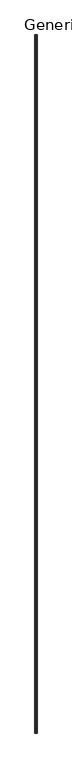
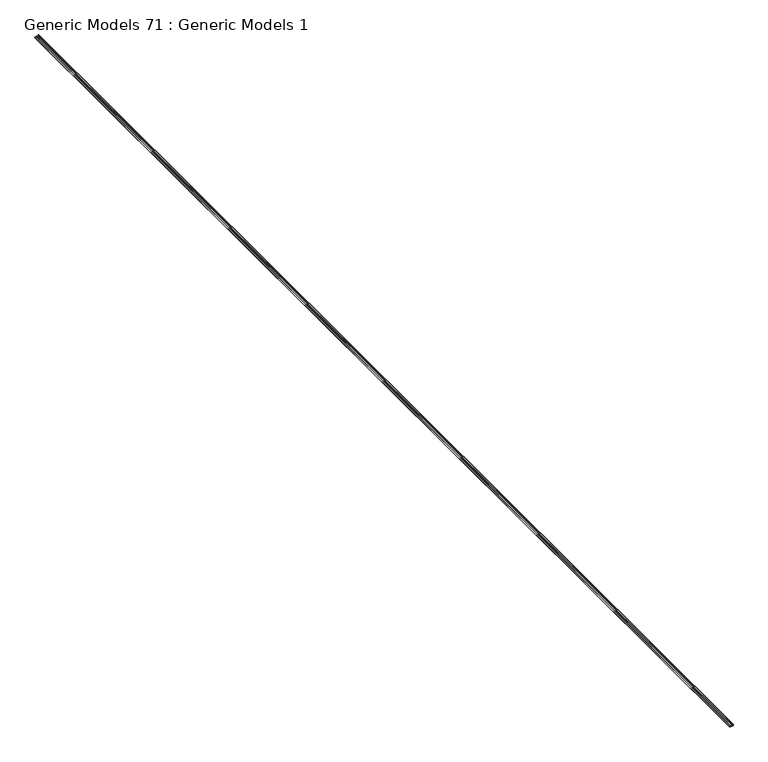
"""IFC4 building model written with IfcOpenShell, lengths in millimetres: proxy geometry, Generic Models 71 : Generic Models 1."""

from ifc_helpers import new_model, si_unit, frame, origin, place, context, project, spatial, polyline, outline, extrude, source, transform, mapped, element, save


def generic_models_71_generic_models_1_deb8e508(model_context):
    return source(origin(), model_context, "Body", "SweptSolid", [
        extrude(outline(polyline([(142822.070303, -9211.2597887), (142822.070303, -9230.9447887), (142833.500303, -9230.9447887), (142833.500303, -9246.1847887), (142822.070303, -9246.1847887), (142822.070303, -9268.6279726), (142820.800303, -9268.6279726), (142820.800303, -9244.9147887), (142832.230303, -9244.9147887), (142832.230303, -9232.2147887), (142820.800303, -9232.2147887), (142820.800303, -9209.9897887), (142825.550103, -9209.9897887), (142825.550103, -9210.8486296), (142844.5946817, -9210.8486296), (142844.5946817, -9212.1186296), (142824.280103, -9212.1186296), (142824.280103, -9211.2597887), (142822.070303, -9211.2597887)])), frame((0.0, -7068.1230338, 0.0), z_axis=(0.0, 1.0, 0.0), x_axis=(0.0, 0.0, 1.0)), (0.0, 0.0, 1.0), 19050.0),
    ])


if __name__ == "__main__":
    model = new_model("IFC4")
    model_context = context("Model", 3, world=origin())
    ifc_project = project(units=[si_unit("LENGTHUNIT", "METRE", prefix="MILLI")], contexts=[model_context])
    site = spatial("IfcSite", under=ifc_project)
    building = spatial("IfcBuilding", under=site)
    placement = place(None, origin())
    generic_models_71_generic_models_1_shape = generic_models_71_generic_models_1_deb8e508(model_context)
    element("IfcBuildingElementProxy", 1, Name="Generic Models 71 : Generic Models 1", ObjectType="Generic Models 71 : Generic Models 1", at=placement, inside=building, context=model_context, shape_type="MappedRepresentation", body=[
        mapped(generic_models_71_generic_models_1_shape, transform((0.0, 0.0, 0.0), x_axis=(1.0, 0.0, 0.0), y_axis=(0.0, 1.0, 0.0), z_axis=(0.0, 0.0, 1.0))),
    ])
    save(model, "model.ifc")

# Revit data of these elements
# Element 1 (IfcBuildingElementProxy, "Generic Models 71 : Generic Models 1")
#   Materials on its faces: "_16 GA. COPPER SOFFIT DRIP SCREED"
# Materials
#   "_16 GA. COPPER SOFFIT DRIP SCREED": class "Generic", colour RGB 253 192 103, transparency 0, Cost = 0
